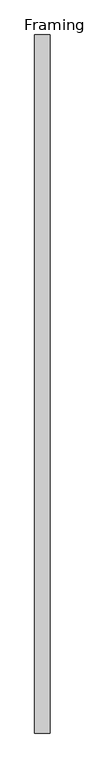
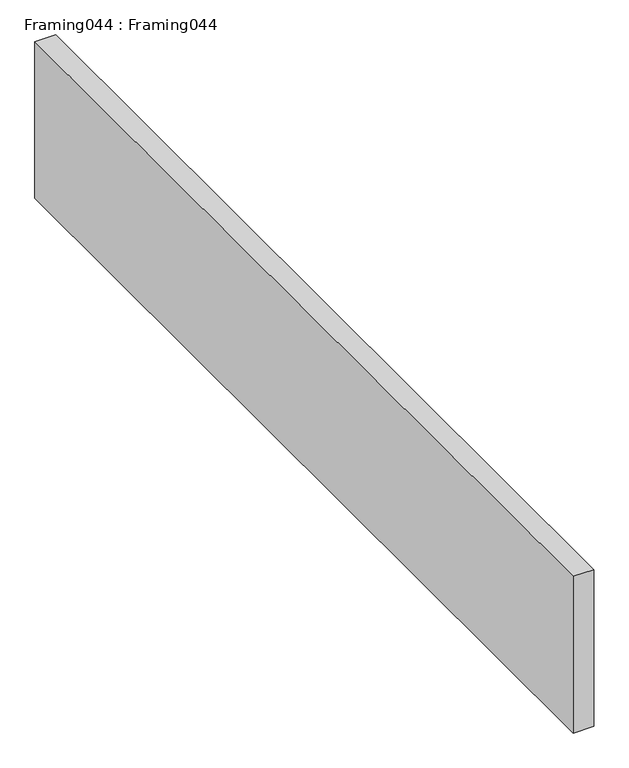
"""IFC4 building model written with IfcOpenShell, lengths in millimetres: proxy geometry, Framing044 : Framing044."""

from ifc_helpers import new_model, si_unit, frame, origin, place, context, project, spatial, polyline, outline, extrude, source, transform, mapped, element, save


def framing044_framing044_f0e99a74(model_context):
    return source(origin(), model_context, "Body", "SweptSolid", [
        extrude(outline(polyline([(-5378.999396, 7982.1531721), (-5423.449396, 7982.1531721), (-5423.449396, 9982.1531721), (-5378.999396, 9982.1531721), (-5378.999396, 7982.1531721)])), frame((0.0, 0.0, 43056.5101822), z_axis=(0.0, 0.0, 1.0), x_axis=(1.0, 0.0, 0.0)), (0.0, 0.0, 1.0), 355.2981173),
    ])


if __name__ == "__main__":
    model = new_model("IFC4")
    model_context = context("Model", 3, world=origin())
    ifc_project = project(units=[si_unit("LENGTHUNIT", "METRE", prefix="MILLI")], contexts=[model_context])
    site = spatial("IfcSite", under=ifc_project)
    building = spatial("IfcBuilding", under=site)
    placement = place(None, origin())
    framing044_framing044_shape = framing044_framing044_f0e99a74(model_context)
    element("IfcBuildingElementProxy", 1, Name="Framing044 : Framing044", ObjectType="Framing044 : Framing044", at=placement, inside=building, context=model_context, shape_type="MappedRepresentation", body=[
        mapped(framing044_framing044_shape, transform((0.0, 0.0, 0.0), x_axis=(1.0, 0.0, 0.0), y_axis=(0.0, 1.0, 0.0), z_axis=(0.0, 0.0, 1.0))),
    ])
    save(model, "model.ifc")

# Revit data of these elements
# Type "Framing044 : Framing044"
#   NameOverride = "Framing044"
# Element 1 (IfcBuildingElementProxy, "Framing044 : Framing044")
#   Materials on its faces: "WOOD FRAMING (SEE STRUCT DWGS)"
# Materials
#   "WOOD FRAMING (SEE STRUCT DWGS)": class "Unassigned", colour RGB 224 188 168, transparency 0, Cost = 0
